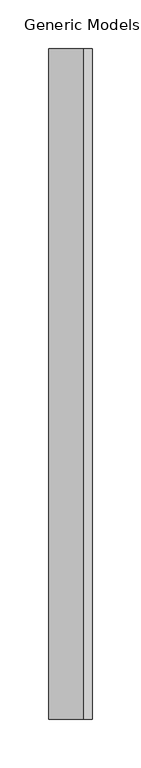
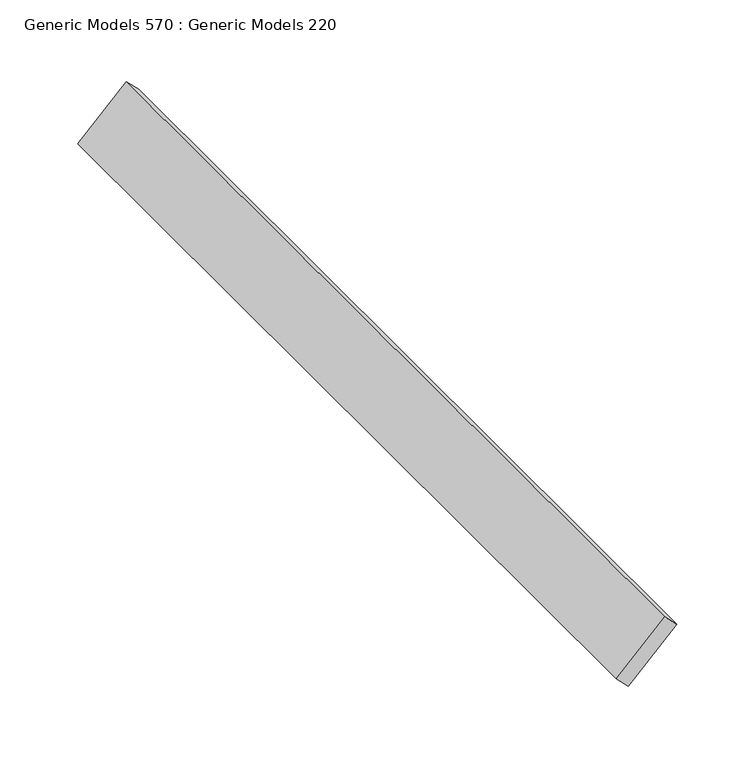
"""IFC4 building model written with IfcOpenShell, lengths in millimetres: proxy geometry, Generic Models 570 : Generic Models 220."""

from ifc_helpers import new_model, si_unit, frame, origin, place, context, project, spatial, polyline, outline, extrude, source, transform, mapped, element, save


def generic_models_570_generic_models_220_7f703335(model_context):
    return source(origin(), model_context, "Body", "SweptSolid", [
        extrude(outline(polyline([(0.0, -12.7000001), (0.0, 0.0), (690.8142348, 0.0), (690.8142348, -12.7000001), (0.0, -12.7000001)])), frame((7841.3059863, 4539.4872686, 124049.1399101), z_axis=(0.7071067811868034, 0.0, 0.7071067811862918), x_axis=(0.0, -1.0, 0.0)), (0.0, 0.0, 1.0), 50.8),
    ])


if __name__ == "__main__":
    model = new_model("IFC4")
    model_context = context("Model", 3, world=origin())
    ifc_project = project(units=[si_unit("LENGTHUNIT", "METRE", prefix="MILLI")], contexts=[model_context])
    site = spatial("IfcSite", under=ifc_project)
    building = spatial("IfcBuilding", under=site)
    placement = place(None, origin())
    generic_models_570_generic_models_220_shape = generic_models_570_generic_models_220_7f703335(model_context)
    element("IfcBuildingElementProxy", 1, Name="Generic Models 570 : Generic Models 220", ObjectType="Generic Models 570 : Generic Models 220", at=placement, inside=building, context=model_context, shape_type="MappedRepresentation", body=[
        mapped(generic_models_570_generic_models_220_shape, transform((0.0, 0.0, 0.0), x_axis=(1.0, 0.0, 0.0), y_axis=(0.0, 1.0, 0.0), z_axis=(0.0, 0.0, 1.0))),
    ])
    save(model, "model.ifc")

# Revit data of these elements
# Element 1 (IfcBuildingElementProxy, "Generic Models 570 : Generic Models 220")
#   Materials on its faces: "_WOOD TONE ALUMINUM EXTRUSION SLAT BY KNOTWOOD"
# Materials
#   "_WOOD TONE ALUMINUM EXTRUSION SLAT BY KNOTWOOD": class "Generic", colour RGB 177 130 114, transparency 0, Cost = 0
